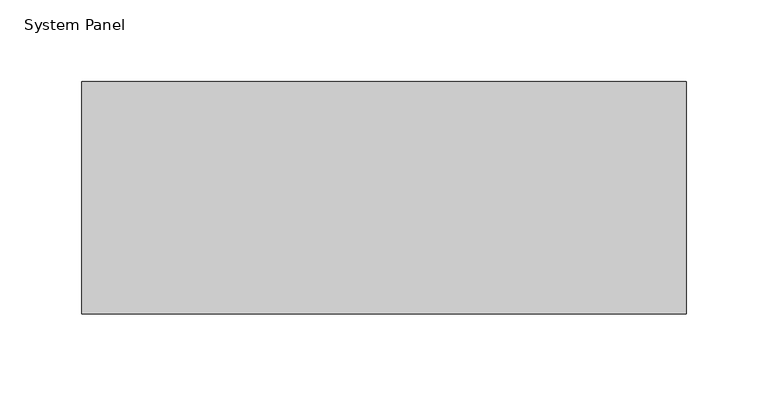
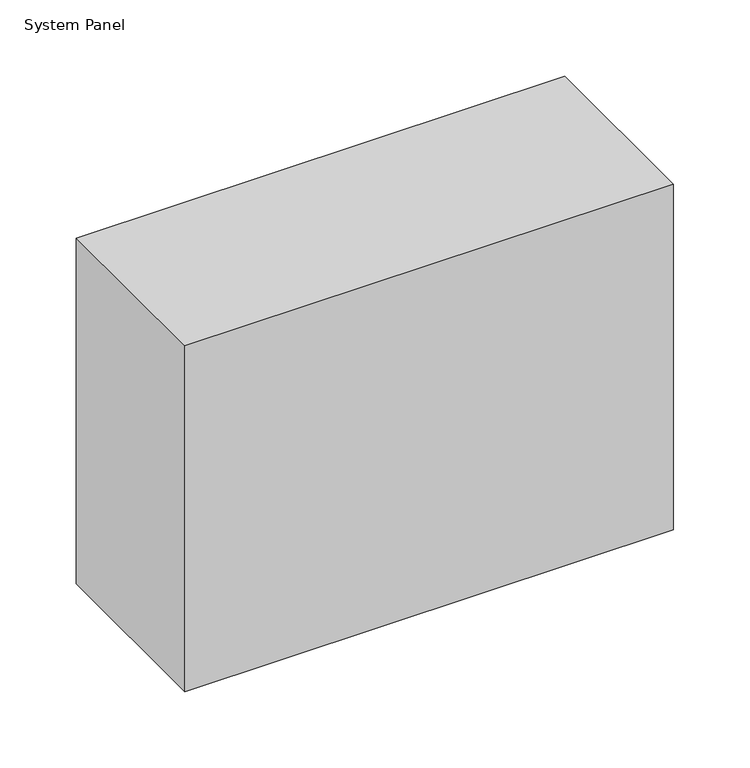
"""IFC4 building model written with IfcOpenShell, lengths in millimetres: plate geometry, System Panel : NLRS_21_CWP_hsb-vulling minerale wol 142 _gen_rsf."""

from ifc_helpers import new_model, si_unit, origin, origin_with_axes, place, context, project, spatial, polyline, outline, extrude, source, transform, mapped, element, save


def system_panel_0d6cc1c8(model_context):
    return source(origin(), model_context, "Body", "SweptSolid", [
        extrude(outline(polyline([(184.5, -71.0), (-184.5, -71.0), (-184.5, 71.0), (184.5, 71.0), (184.5, -71.0)])), origin_with_axes(), (0.0, 0.0, 1.0), 276.0),
    ])


if __name__ == "__main__":
    model = new_model("IFC4")
    model_context = context("Model", 3, world=origin())
    ifc_project = project(units=[si_unit("LENGTHUNIT", "METRE", prefix="MILLI")], contexts=[model_context])
    site = spatial("IfcSite", under=ifc_project)
    building = spatial("IfcBuilding", under=site)
    placement = place(None, origin())
    system_panel_shape = system_panel_0d6cc1c8(model_context)
    element("IfcPlate", 1, ObjectType="System Panel : NLRS_21_CWP_hsb-vulling minerale wol 142 _gen_rsf", at=placement, inside=building, context=model_context, shape_type="MappedRepresentation", body=[
        mapped(system_panel_shape, transform((0.0, 0.0, 0.0), x_axis=(1.0, 0.0, 0.0), y_axis=(0.0, 1.0, 0.0), z_axis=(0.0, 0.0, 1.0))),
    ])
    save(model, "model.ifc")

# Revit data of these elements
# Type "System Panel : NLRS_21_CWP_hsb-vulling minerale wol 142 _gen_rsf"
#   Export Type to IFC As = "IfcWall"
#   Type IfcGUID = "07M7mRoiH1CR8m_RSKIwpC"
#   Assembly Code = "21.23"
# Element 1 (IfcPlate, "System Panel : NLRS_21_CWP_hsb-vulling minerale wol 142 _gen_rsf")
#   Materials on its faces: "NLRS_m1_isolatie minerale wol_gen_rsf"
# Materials
#   "NLRS_m1_isolatie minerale wol_gen_rsf": class "M - Anorganische materialen", colour RGB 200 200 140, transparency 0, Keynote = "m1", Manufacturer = "Revit Standards Foundation", URL = "www.revitstandards.org", Description = "isolatie minerale wol", Cost = 0
